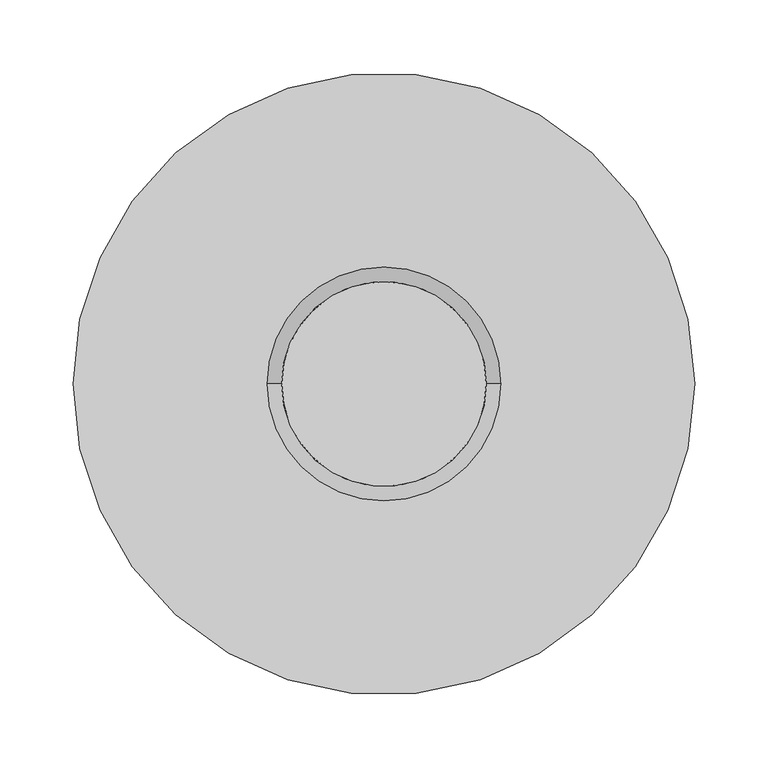
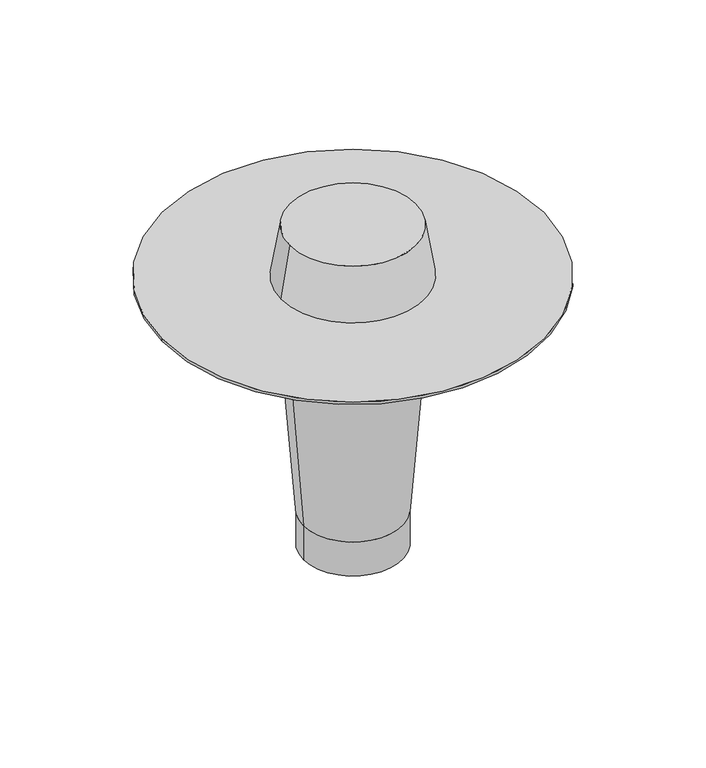
"""IFC4 building model written with IfcOpenShell, lengths in millimetres: proxy geometry, TN_Воронка ТехноНИКОЛЬ ВБ : Воронка ТехноНИКОЛЬ ВБ ЭКО, 110х315."""

from ifc_helpers import new_model, si_unit, point, frame, origin, origin_2d, place, context, project, spatial, polyline, circle_curve, trimmed, segment, composite_curve, outline, extrude, source, transform, mapped, element, save
from ifc_brep_helpers import plane_surface, revolved_surface, advanced_brep


def specialty_equipment_fed2c7da(model_context):
    return source(origin(), model_context, "Body", "SolidModel", [
        advanced_brep(
        [(70.0, 0.0, -85.0), (-70.0, 0.0, -85.0), (55.0, 0.0, -275.0), (-55.0, 0.0, -275.0)],
        [
            (0, 1, circle_curve(frame((0.0, 0.0, -85.0), z_axis=(0.0, 0.0, 1.0), x_axis=(1.0, 0.0, 0.0)), 70.0)),
            (1, 0, circle_curve(frame((0.0, 0.0, -85.0), z_axis=(0.0, 0.0, 1.0), x_axis=(-1.0, 0.0, 0.0)), 70.0)),
            (2, 3, circle_curve(frame((0.0, 0.0, -275.0), z_axis=(0.0, 0.0, -1.0), x_axis=(-1.0, 0.0, 0.0)), 55.0)),
            (3, 2, circle_curve(frame((0.0, 0.0, -275.0), z_axis=(0.0, 0.0, -1.0), x_axis=(1.0, 0.0, 0.0)), 55.0)),
            (3, 1),
            (0, 2),
        ],
        [
            plane_surface(frame((0.0, 0.0, -85.0), z_axis=(0.0, 0.0, 1.0), x_axis=(0.0, 1.0, 0.0))),
            plane_surface(frame((0.0, 0.0, -275.0), z_axis=(0.0, 0.0, -1.0), x_axis=(0.0, 1.0, 0.0))),
            revolved_surface(polyline([(-55.00000000056391, 0.0, -275.0), (-70.0, 0.0, -85.0)]), (0.0, 0.0, -971.6666667), (0.0, 0.0, 1.0)),
            revolved_surface(polyline([(55.00000000056391, 0.0, -275.0), (70.0, 0.0, -85.0)]), (0.0, 0.0, -971.6666667), (0.0, 0.0, 1.0)),
        ],
        [
            (0, [[1, 2]]),
            (1, [[3, 4]]),
            (2, [[-4, 5, -1, 6]]),
            (3, [[-3, -6, -2, -5]]),
        ],
    ),
        extrude(outline(composite_curve([segment(trimmed(circle_curve(origin_2d(), 70.0), [point((-70.0, 0.0))], [point((70.0, 0.0))], False, "CARTESIAN"), True, "CONTINUOUS"), segment(trimmed(circle_curve(origin_2d(), 70.0), [point((70.0, 0.0))], [point((-70.0, 0.0))], False, "CARTESIAN"), True, "CONTINUOUS")], self_intersect=False)), frame((0.0, 0.0, -85.0), z_axis=(0.0, 0.0, 1.0), x_axis=(1.0, 0.0, 0.0)), (0.0, 0.0, 1.0), 82.0),
        extrude(outline(composite_curve([segment(trimmed(circle_curve(origin_2d(), 55.0), [point((55.0, 0.0))], [point((-55.0, 0.0))], False, "CARTESIAN"), True, "CONTINUOUS"), segment(trimmed(circle_curve(origin_2d(), 55.0), [point((-55.0, 0.0))], [point((55.0, 0.0))], False, "CARTESIAN"), True, "CONTINUOUS")], self_intersect=False)), frame((0.0, 0.0, -315.0), z_axis=(0.0, 0.0, 1.0), x_axis=(1.0, 0.0, 0.0)), (0.0, 0.0, 1.0), 40.0),
        extrude(outline(composite_curve([segment(trimmed(circle_curve(origin_2d(), 212.5), [point((-212.5, 0.0))], [point((212.5, 0.0))], False, "CARTESIAN"), True, "CONTINUOUS"), segment(trimmed(circle_curve(origin_2d(), 212.5), [point((212.5, 0.0))], [point((-212.5, 0.0))], False, "CARTESIAN"), True, "CONTINUOUS")], self_intersect=False)), frame((0.0, 0.0, -3.0), z_axis=(0.0, 0.0, 1.0), x_axis=(1.0, 0.0, 0.0)), (0.0, 0.0, 1.0), 3.0),
        advanced_brep(
        [(-70.0, 0.0, 60.0), (70.0, 0.0, 60.0), (-80.0, 0.0, 0.0), (80.0, 0.0, 0.0)],
        [
            (0, 1, circle_curve(frame((0.0, 0.0, 60.0), z_axis=(0.0, 0.0, 1.0), x_axis=(-1.0, 0.0, 0.0)), 70.0)),
            (1, 0, circle_curve(frame((0.0, 0.0, 60.0), z_axis=(0.0, 0.0, 1.0), x_axis=(1.0, 0.0, 0.0)), 70.0)),
            (2, 3, circle_curve(frame((0.0, 0.0, 0.0), z_axis=(0.0, 0.0, -1.0), x_axis=(1.0, 0.0, 0.0)), 80.0)),
            (3, 2, circle_curve(frame((0.0, 0.0, 0.0), z_axis=(0.0, 0.0, -1.0), x_axis=(-1.0, 0.0, 0.0)), 80.0)),
            (3, 1),
            (0, 2),
        ],
        [
            plane_surface(frame((0.0, 0.0, 60.0), z_axis=(0.0, 0.0, 1.0), x_axis=(0.0, -1.0, 0.0))),
            plane_surface(frame((0.0, 0.0, 0.0), z_axis=(0.0, 0.0, -1.0), x_axis=(0.0, -1.0, 0.0))),
            revolved_surface(polyline([(-70.0, 0.0, 60.0), (-80.0, 0.0, 0.0)]), (0.0, 0.0, 480.0), (0.0, 0.0, -1.0)),
            revolved_surface(polyline([(70.0, 0.0, 60.0), (80.0, 0.0, 0.0)]), (0.0, 0.0, 480.0), (0.0, 0.0, -1.0)),
        ],
        [
            (0, [[1, 2]]),
            (1, [[3, 4]]),
            (2, [[-4, 5, -1, 6]]),
            (3, [[-3, -6, -2, -5]]),
        ],
    ),
    ])


if __name__ == "__main__":
    model = new_model("IFC4")
    model_context = context("Model", 3, world=origin())
    ifc_project = project(units=[si_unit("LENGTHUNIT", "METRE", prefix="MILLI")], contexts=[model_context])
    site = spatial("IfcSite", under=ifc_project)
    building = spatial("IfcBuilding", under=site)
    placement = place(None, origin())
    specialty_equipment_shape = specialty_equipment_fed2c7da(model_context)
    element("IfcBuildingElementProxy", 1, Name="TN_Воронка ТехноНИКОЛЬ ВБ : Воронка ТехноНИКОЛЬ ВБ ЭКО, 110х315", ObjectType="TN_Воронка ТехноНИКОЛЬ ВБ : Воронка ТехноНИКОЛЬ ВБ ЭКО, 110х315", at=placement, inside=building, context=model_context, shape_type="MappedRepresentation", body=[
        mapped(specialty_equipment_shape, transform((0.0, 0.0, 0.0), x_axis=(1.0, 0.0, 0.0), y_axis=(0.0, 1.0, 0.0), z_axis=(0.0, 0.0, 1.0))),
    ])
    save(model, "model.ifc")

# Revit data of these elements
# Type "TN_Воронка ТехноНИКОЛЬ ВБ : Воронка ТехноНИКОЛЬ ВБ ЭКО, 110х315"
#   ADSK_Группирование = "Комплектующие и воронки"
#   Description = "Кровельные воронки ТехноНИКОЛЬ ВБ ЭКО 110х315 применяются для организации внутреннего водостока с плоских кровель. Воронки могут устанавливаться в кровлю безогневым способом на мастику герметизирующую № 71. Воронки ТехноНИКОЛЬ ВБ ЭКО 110х315 используются при ремонте и строительстве зданий и сооружений с плоскими кровлями. Применяются в кровлях из битумных и битумнополимерных рулонных и мастичных материалов с внутренним водостоком. Количество воронок определяется расчетом. Пропуская способность 7,8 л/сек."
#   Manufacturer = "ТехноНИКОЛЬ"
#   URL = "https://shop.tn.ru/voronka-tehnonikol-vb-jeko-110h315-mm"
#   ADSK_Примечание = ""
#   ADSK_Обозначение = "ТехноНИКОЛЬ"
#   ADSK_Наименование = "Воронка ТехноНИКОЛЬ ВБ ЭКО, 110х315"
#   ADSK_Марка = ""
#   ADSK_Код изделия = "460067"
#   ADSK_Завод-изготовитель = "ТехноНИКОЛЬ"
#   ADSK_Единица измерения = "шт."
#   ADSK_Группирование = "Комплектующие и воронки"
#   ADSK_URL страницы изделия = "https://shop.tn.ru/voronka-tehnonikol-vb-jeko-110h315-mm"
#   ADSK_URL документации изделия = "https://nav.tn.ru/catalog/krovlya/vodostochnaya-sistema/voronka-tekhnonikol-vb-eko/?sphrase_id=114614"
#   Диаметр фланца = 425 mm
#   Высота воронки = 315 mm
#   ADSK_Масса = 0.6
#   ADSK_Количество = 1
#   Материал = TN_ПВХ_Черный
#   Default Elevation = 0
# Element 1 (IfcBuildingElementProxy, "TN_Воронка ТехноНИКОЛЬ ВБ : Воронка ТехноНИКОЛЬ ВБ ЭКО, 110х315")
#   Materials on its faces: "TN_ПВХ_Черный"
# Materials
#   "TN_ПВХ_Черный": class "Типовые", colour RGB 48 48 48, transparency 0, Cost = 0
